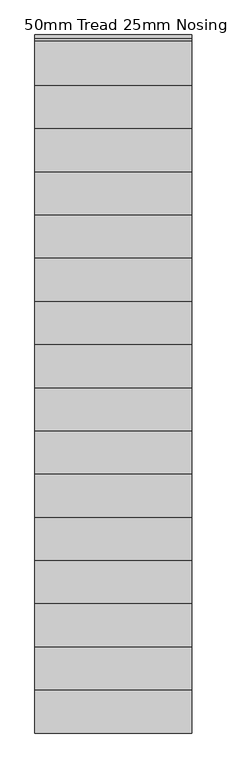
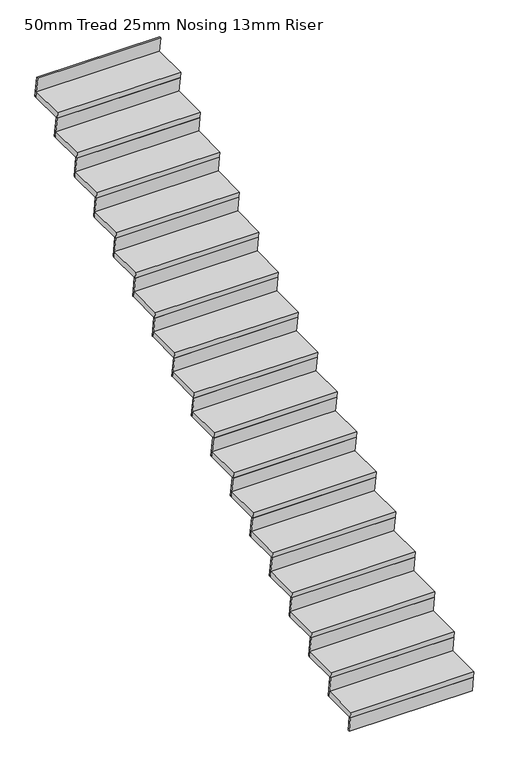
"""IFC4 building model written with IfcOpenShell, lengths in millimetres: stair flight geometry, 50mm Tread 25mm Nosing 13mm Riser."""

import ifcopenshell
import ifcopenshell.guid

model = None  # the IFC model being written
_history = None  # IfcOwnerHistory: only IFC2X3 demands one
_inside = {}  # id of a spatial element -> (the spatial element, [elements in it])
_under = {}  # id of a project, library or spatial element -> (it, [spatial elements below it])
_declared = {}  # id of a project -> (the project, [libraries it declares])
_typed = {}  # id of a type object -> (the type object, [elements of that type])
_made_of = {}  # id of a material, layer set ... -> (it, [elements and type objects made of it])


def new_model(schema):
    """Start an empty IFC model of exactly this schema.

    Asked for "IFC4X3", IfcOpenShell would pick the latest addendum, in which some entities
    have other attributes; the version numbers below select the first issue.
    IFC2X3 requires an IfcOwnerHistory on every rooted entity: one is made here for all.
    """
    global model, _history
    if schema == "IFC4X3":
        model = ifcopenshell.file(schema_version=(4, 3, 0, 0))
    else:
        model = ifcopenshell.file(schema=schema)
    _inside.clear()
    _under.clear()
    _declared.clear()
    _typed.clear()
    _made_of.clear()
    _history = None
    if model.schema == "IFC2X3":
        org = make("IfcOrganization", Name="unknown")
        user = make(
            "IfcPersonAndOrganization",
            ThePerson=make("IfcPerson", FamilyName="unknown"),
            TheOrganization=org,
        )
        app = make(
            "IfcApplication",
            ApplicationDeveloper=org,
            Version="unknown",
            ApplicationFullName="unknown",
            ApplicationIdentifier="unknown",
        )
        _history = make(
            "IfcOwnerHistory",
            OwningUser=user,
            OwningApplication=app,
            ChangeAction="ADDED",
            CreationDate=0,
        )
    return model


def make(cls, **values):
    """One entity of the class cls with the attributes given. An attribute that is None is left unset."""
    return model.create_entity(
        cls, **{name: value for name, value in values.items() if value is not None}
    )


def rooted(cls, **values):
    """An entity with a GlobalId (a new one), such as an element, a storey or a relation."""
    return make(cls, GlobalId=ifcopenshell.guid.new(), OwnerHistory=_history, **values)


def si_unit(unit_type, name, prefix=None):
    """IfcSIUnit, for example si_unit("LENGTHUNIT", "METRE", prefix="MILLI")."""
    return make("IfcSIUnit", UnitType=unit_type, Prefix=prefix, Name=name)


def assignment(units):
    """IfcUnitAssignment: the units of a project."""
    return None if units is None else make("IfcUnitAssignment", Units=units)


def point(xyz):
    """IfcCartesianPoint."""
    return None if xyz is None else make("IfcCartesianPoint", Coordinates=xyz)


def direction(xyz):
    """IfcDirection."""
    return None if xyz is None else make("IfcDirection", DirectionRatios=xyz)


def frame(location, z_axis=None, x_axis=None):
    """IfcAxis2Placement3D, a coordinate frame: its origin and axes. An axis left out is left unset."""
    return make(
        "IfcAxis2Placement3D",
        Location=point(location),
        Axis=direction(z_axis),
        RefDirection=direction(x_axis),
    )


def origin():
    """The frame at (0, 0, 0) with its axes left unset."""
    return frame((0.0, 0.0, 0.0))


def place(relative_to, where):
    """IfcLocalPlacement: puts the frame where relative to a parent placement (None: the world)."""
    return make(
        "IfcLocalPlacement", PlacementRelTo=relative_to, RelativePlacement=where
    )


def context(
    kind, dimensions, precision=None, world=None, true_north=None, identifier=None
):
    """IfcGeometricRepresentationContext, for example the 3D "Model" context."""
    return make(
        "IfcGeometricRepresentationContext",
        ContextIdentifier=identifier,
        ContextType=kind,
        CoordinateSpaceDimension=dimensions,
        Precision=precision,
        WorldCoordinateSystem=world,
        TrueNorth=true_north,
    )


def project(units=None, contexts=None):
    """IfcProject with its units and contexts."""
    return rooted(
        "IfcProject",
        Name="project",
        RepresentationContexts=contexts,
        UnitsInContext=assignment(units),
    )


def spatial(cls, under=None, at=None, **own):
    """A site, building, storey or space (cls), placed at a placement, below another one or the project."""
    s = rooted(cls, ObjectPlacement=at, **own)
    if under is not None:
        _under.setdefault(under.id(), (under, []))[1].append(s)
    return s


def polyline(points):
    """IfcPolyline through the points."""
    return make("IfcPolyline", Points=[point(p) for p in points])


def outline(outer, holes=None, kind="AREA"):
    """IfcArbitraryClosedProfileDef: a profile drawn as a closed curve; with holes, ...WithVoids."""
    if holes is None:
        return make("IfcArbitraryClosedProfileDef", ProfileType=kind, OuterCurve=outer)
    return make(
        "IfcArbitraryProfileDefWithVoids",
        ProfileType=kind,
        OuterCurve=outer,
        InnerCurves=holes,
    )


def extrude(swept, where, along, depth):
    """IfcExtrudedAreaSolid: the profile swept, set in the frame where, extruded along a direction by depth."""
    return make(
        "IfcExtrudedAreaSolid",
        SweptArea=swept,
        Position=where,
        ExtrudedDirection=direction(along),
        Depth=depth,
    )


def shape(context_of_items, identifier, shape_type, items):
    """IfcShapeRepresentation: the items that make up one representation, for example the "Body"."""
    return make(
        "IfcShapeRepresentation",
        ContextOfItems=context_of_items,
        RepresentationIdentifier=identifier,
        RepresentationType=shape_type,
        Items=items,
    )


def source(mapping_origin, context_of_items, identifier, shape_type, items):
    """IfcRepresentationMap: a shape defined once, which mapped items show again and again."""
    return make(
        "IfcRepresentationMap",
        MappingOrigin=mapping_origin,
        MappedRepresentation=shape(context_of_items, identifier, shape_type, items),
    )


def transform(
    local_origin,
    x_axis=None,
    y_axis=None,
    z_axis=None,
    scale=None,
    scale2=None,
    scale3=None,
    uniform=True,
):
    """IfcCartesianTransformationOperator3D, or its non-uniform kind. x_axis, y_axis, z_axis: its Axis1, 2, 3."""
    if uniform:
        return make(
            "IfcCartesianTransformationOperator3D",
            Axis1=direction(x_axis),
            Axis2=direction(y_axis),
            LocalOrigin=point(local_origin),
            Scale=scale,
            Axis3=direction(z_axis),
        )
    return make(
        "IfcCartesianTransformationOperator3DnonUniform",
        Axis1=direction(x_axis),
        Axis2=direction(y_axis),
        LocalOrigin=point(local_origin),
        Scale=scale,
        Axis3=direction(z_axis),
        Scale2=scale2,
        Scale3=scale3,
    )


def mapped(mapping_source, mapping_target):
    """IfcMappedItem: shows the shape of a source again, moved by a transform."""
    return make(
        "IfcMappedItem", MappingSource=mapping_source, MappingTarget=mapping_target
    )


def made_of(thing, what):
    """Note that an element or type object is made of a material, layer set ...; save() writes the relation."""
    if what is not None:
        _made_of.setdefault(what.id(), (what, []))[1].append(thing)
    return thing


def element(
    cls,
    number,
    at=None,
    inside=None,
    cuts=None,
    type_object=None,
    material=None,
    context=None,
    identifier="Body",
    shape_type=None,
    held_by="IfcProductDefinitionShape",
    body=None,
    shapes=None,
    **own,
):
    """One element of the class cls, such as IfcWall. Its Tag is "e" and its number.

    at: its placement. inside: the storey or other place that contains it. cuts: it is an
    opening in that element (IfcRelVoidsElement). A single representation is given by context,
    identifier, shape_type and body (its items); several are given by shapes. held_by: the class
    of the entity that holds the representations. save() writes the other relations.
    """
    e = rooted(cls, Tag="e%d" % number, ObjectPlacement=at, **own)
    if body is not None:
        shapes = [shape(context, identifier, shape_type, body)]
    if shapes is not None:
        e.Representation = make(held_by, Representations=shapes)
    if inside is not None:
        _inside.setdefault(inside.id(), (inside, []))[1].append(e)
    if cuts is not None:
        rooted(
            "IfcRelVoidsElement", RelatingBuildingElement=cuts, RelatedOpeningElement=e
        )
    if type_object is not None:
        _typed.setdefault(type_object.id(), (type_object, []))[1].append(e)
    return made_of(e, material)


def aggregate(whole, parts):
    """IfcRelAggregates: a whole, such as a stair, and the parts it consists of."""
    return rooted("IfcRelAggregates", RelatingObject=whole, RelatedObjects=parts)


def save(model, path):
    """Write the relations noted so far, then the file.

    IfcRelAggregates (storeys below a building ...), IfcRelContainedInSpatialStructure (elements
    in a storey), IfcRelDefinesByType, IfcRelAssociatesMaterial and IfcRelDeclares: one each for
    every whole, place, type object, material and project.
    """
    for whole, parts in _under.values():
        aggregate(whole, parts)
    for where, things in _inside.values():
        rooted(
            "IfcRelContainedInSpatialStructure",
            RelatedElements=things,
            RelatingStructure=where,
        )
    for kind, things in _typed.values():
        rooted("IfcRelDefinesByType", RelatedObjects=things, RelatingType=kind)
    for what, things in _made_of.values():
        rooted("IfcRelAssociatesMaterial", RelatedObjects=things, RelatingMaterial=what)
    for by, libraries in _declared.values():
        rooted("IfcRelDeclares", RelatingContext=by, RelatedDefinitions=libraries)
    model.write(path)


def stair_flight_50mm_tread_25mm_nosing_13mm_riser_3b40119f(model_context):
    return source(origin(), model_context, "Body", "SweptSolid", [
        extrude(outline(polyline([(-31126.6946949, 176.4705882), (-30826.6946949, 176.4705882), (-30819.6113616, 126.4705882), (-31119.6113616, 126.4705882), (-31126.6946949, 176.4705882)])), frame((121318.8827039, 0.0, 0.0), z_axis=(1.0, 0.0, 0.0), x_axis=(0.0, 1.0, 0.0)), (0.0, 0.0, 1.0), 1000.0),
        extrude(outline(polyline([(-31119.6113616, 126.4705882), (-31106.9865507, 126.4705882), (-31089.069884, 0.0), (-31101.6946949, 0.0), (-31119.6113616, 126.4705882)])), frame((121318.8827039, 0.0, 0.0), z_axis=(1.0, 0.0, 0.0), x_axis=(0.0, 1.0, 0.0)), (0.0, 0.0, 1.0), 1000.0),
        extrude(outline(polyline([(-30844.6113616, 302.9411765), (-30831.9865507, 302.9411765), (-30806.9865507, 126.4705882), (-30819.6113616, 126.4705882), (-30844.6113616, 302.9411765)])), frame((121318.8827039, 0.0, 0.0), z_axis=(1.0, 0.0, 0.0), x_axis=(0.0, 1.0, 0.0)), (0.0, 0.0, 1.0), 1000.0),
        extrude(outline(polyline([(-30851.6946949, 352.9411765), (-30551.6946949, 352.9411765), (-30544.6113616, 302.9411765), (-30844.6113616, 302.9411765), (-30851.6946949, 352.9411765)])), frame((121318.8827039, 0.0, 0.0), z_axis=(1.0, 0.0, 0.0), x_axis=(0.0, 1.0, 0.0)), (0.0, 0.0, 1.0), 1000.0),
        extrude(outline(polyline([(-30569.6113616, 479.4117647), (-30556.9865507, 479.4117647), (-30531.9865507, 302.9411765), (-30544.6113616, 302.9411765), (-30569.6113616, 479.4117647)])), frame((121318.8827039, 0.0, 0.0), z_axis=(1.0, 0.0, 0.0), x_axis=(0.0, 1.0, 0.0)), (0.0, 0.0, 1.0), 1000.0),
        extrude(outline(polyline([(-30576.6946949, 529.4117647), (-30276.6946949, 529.4117647), (-30269.6113616, 479.4117647), (-30569.6113616, 479.4117647), (-30576.6946949, 529.4117647)])), frame((121318.8827039, 0.0, 0.0), z_axis=(1.0, 0.0, 0.0), x_axis=(0.0, 1.0, 0.0)), (0.0, 0.0, 1.0), 1000.0),
        extrude(outline(polyline([(-30294.6113616, 655.8823529), (-30281.9865507, 655.8823529), (-30256.9865507, 479.4117647), (-30269.6113616, 479.4117647), (-30294.6113616, 655.8823529)])), frame((121318.8827039, 0.0, 0.0), z_axis=(1.0, 0.0, 0.0), x_axis=(0.0, 1.0, 0.0)), (0.0, 0.0, 1.0), 1000.0),
        extrude(outline(polyline([(-30301.6946949, 705.8823529), (-30001.6946949, 705.8823529), (-29994.6113616, 655.8823529), (-30294.6113616, 655.8823529), (-30301.6946949, 705.8823529)])), frame((121318.8827039, 0.0, 0.0), z_axis=(1.0, 0.0, 0.0), x_axis=(0.0, 1.0, 0.0)), (0.0, 0.0, 1.0), 1000.0),
        extrude(outline(polyline([(-30019.6113616, 832.3529412), (-30006.9865507, 832.3529412), (-29981.9865507, 655.8823529), (-29994.6113616, 655.8823529), (-30019.6113616, 832.3529412)])), frame((121318.8827039, 0.0, 0.0), z_axis=(1.0, 0.0, 0.0), x_axis=(0.0, 1.0, 0.0)), (0.0, 0.0, 1.0), 1000.0),
        extrude(outline(polyline([(-30026.6946949, 882.3529412), (-29726.6946949, 882.3529412), (-29719.6113616, 832.3529412), (-30019.6113616, 832.3529412), (-30026.6946949, 882.3529412)])), frame((121318.8827039, 0.0, 0.0), z_axis=(1.0, 0.0, 0.0), x_axis=(0.0, 1.0, 0.0)), (0.0, 0.0, 1.0), 1000.0),
        extrude(outline(polyline([(-29744.6113616, 1008.8235294), (-29731.9865507, 1008.8235294), (-29706.9865507, 832.3529412), (-29719.6113616, 832.3529412), (-29744.6113616, 1008.8235294)])), frame((121318.8827039, 0.0, 0.0), z_axis=(1.0, 0.0, 0.0), x_axis=(0.0, 1.0, 0.0)), (0.0, 0.0, 1.0), 1000.0),
        extrude(outline(polyline([(-29751.6946949, 1058.8235294), (-29451.6946949, 1058.8235294), (-29444.6113616, 1008.8235294), (-29744.6113616, 1008.8235294), (-29751.6946949, 1058.8235294)])), frame((121318.8827039, 0.0, 0.0), z_axis=(1.0, 0.0, 0.0), x_axis=(0.0, 1.0, 0.0)), (0.0, 0.0, 1.0), 1000.0),
        extrude(outline(polyline([(-29469.6113616, 1185.2941176), (-29456.9865507, 1185.2941176), (-29431.9865507, 1008.8235294), (-29444.6113616, 1008.8235294), (-29469.6113616, 1185.2941176)])), frame((121318.8827039, 0.0, 0.0), z_axis=(1.0, 0.0, 0.0), x_axis=(0.0, 1.0, 0.0)), (0.0, 0.0, 1.0), 1000.0),
        extrude(outline(polyline([(-29476.6946949, 1235.2941176), (-29176.6946949, 1235.2941176), (-29169.6113616, 1185.2941176), (-29469.6113616, 1185.2941176), (-29476.6946949, 1235.2941176)])), frame((121318.8827039, 0.0, 0.0), z_axis=(1.0, 0.0, 0.0), x_axis=(0.0, 1.0, 0.0)), (0.0, 0.0, 1.0), 1000.0),
        extrude(outline(polyline([(-29194.6113616, 1361.7647059), (-29181.9865507, 1361.7647059), (-29156.9865507, 1185.2941176), (-29169.6113616, 1185.2941176), (-29194.6113616, 1361.7647059)])), frame((121318.8827039, 0.0, 0.0), z_axis=(1.0, 0.0, 0.0), x_axis=(0.0, 1.0, 0.0)), (0.0, 0.0, 1.0), 1000.0),
        extrude(outline(polyline([(-29201.6946949, 1411.7647059), (-28901.6946949, 1411.7647059), (-28894.6113616, 1361.7647059), (-29194.6113616, 1361.7647059), (-29201.6946949, 1411.7647059)])), frame((121318.8827039, 0.0, 0.0), z_axis=(1.0, 0.0, 0.0), x_axis=(0.0, 1.0, 0.0)), (0.0, 0.0, 1.0), 1000.0),
        extrude(outline(polyline([(-28919.6113616, 1538.2352941), (-28906.9865507, 1538.2352941), (-28881.9865507, 1361.7647059), (-28894.6113616, 1361.7647059), (-28919.6113616, 1538.2352941)])), frame((121318.8827039, 0.0, 0.0), z_axis=(1.0, 0.0, 0.0), x_axis=(0.0, 1.0, 0.0)), (0.0, 0.0, 1.0), 1000.0),
        extrude(outline(polyline([(-28926.6946949, 1588.2352941), (-28626.6946949, 1588.2352941), (-28619.6113616, 1538.2352941), (-28919.6113616, 1538.2352941), (-28926.6946949, 1588.2352941)])), frame((121318.8827039, 0.0, 0.0), z_axis=(1.0, 0.0, 0.0), x_axis=(0.0, 1.0, 0.0)), (0.0, 0.0, 1.0), 1000.0),
        extrude(outline(polyline([(-28644.6113616, 1714.7058824), (-28631.9865507, 1714.7058824), (-28606.9865507, 1538.2352941), (-28619.6113616, 1538.2352941), (-28644.6113616, 1714.7058824)])), frame((121318.8827039, 0.0, 0.0), z_axis=(1.0, 0.0, 0.0), x_axis=(0.0, 1.0, 0.0)), (0.0, 0.0, 1.0), 1000.0),
        extrude(outline(polyline([(-28651.6946949, 1764.7058824), (-28351.6946949, 1764.7058824), (-28344.6113616, 1714.7058824), (-28644.6113616, 1714.7058824), (-28651.6946949, 1764.7058824)])), frame((121318.8827039, 0.0, 0.0), z_axis=(1.0, 0.0, 0.0), x_axis=(0.0, 1.0, 0.0)), (0.0, 0.0, 1.0), 1000.0),
        extrude(outline(polyline([(-28369.6113616, 1891.1764706), (-28356.9865507, 1891.1764706), (-28331.9865507, 1714.7058824), (-28344.6113616, 1714.7058824), (-28369.6113616, 1891.1764706)])), frame((121318.8827039, 0.0, 0.0), z_axis=(1.0, 0.0, 0.0), x_axis=(0.0, 1.0, 0.0)), (0.0, 0.0, 1.0), 1000.0),
        extrude(outline(polyline([(-28376.6946949, 1941.1764706), (-28076.6946949, 1941.1764706), (-28069.6113616, 1891.1764706), (-28369.6113616, 1891.1764706), (-28376.6946949, 1941.1764706)])), frame((121318.8827039, 0.0, 0.0), z_axis=(1.0, 0.0, 0.0), x_axis=(0.0, 1.0, 0.0)), (0.0, 0.0, 1.0), 1000.0),
        extrude(outline(polyline([(-28094.6113616, 2067.6470588), (-28081.9865507, 2067.6470588), (-28056.9865507, 1891.1764706), (-28069.6113616, 1891.1764706), (-28094.6113616, 2067.6470588)])), frame((121318.8827039, 0.0, 0.0), z_axis=(1.0, 0.0, 0.0), x_axis=(0.0, 1.0, 0.0)), (0.0, 0.0, 1.0), 1000.0),
        extrude(outline(polyline([(-28101.6946949, 2117.6470588), (-27801.6946949, 2117.6470588), (-27794.6113616, 2067.6470588), (-28094.6113616, 2067.6470588), (-28101.6946949, 2117.6470588)])), frame((121318.8827039, 0.0, 0.0), z_axis=(1.0, 0.0, 0.0), x_axis=(0.0, 1.0, 0.0)), (0.0, 0.0, 1.0), 1000.0),
        extrude(outline(polyline([(-27819.6113616, 2244.1176471), (-27806.9865507, 2244.1176471), (-27781.9865507, 2067.6470588), (-27794.6113616, 2067.6470588), (-27819.6113616, 2244.1176471)])), frame((121318.8827039, 0.0, 0.0), z_axis=(1.0, 0.0, 0.0), x_axis=(0.0, 1.0, 0.0)), (0.0, 0.0, 1.0), 1000.0),
        extrude(outline(polyline([(-27826.6946949, 2294.1176471), (-27526.6946949, 2294.1176471), (-27519.6113616, 2244.1176471), (-27819.6113616, 2244.1176471), (-27826.6946949, 2294.1176471)])), frame((121318.8827039, 0.0, 0.0), z_axis=(1.0, 0.0, 0.0), x_axis=(0.0, 1.0, 0.0)), (0.0, 0.0, 1.0), 1000.0),
        extrude(outline(polyline([(-27544.6113616, 2420.5882353), (-27531.9865507, 2420.5882353), (-27506.9865507, 2244.1176471), (-27519.6113616, 2244.1176471), (-27544.6113616, 2420.5882353)])), frame((121318.8827039, 0.0, 0.0), z_axis=(1.0, 0.0, 0.0), x_axis=(0.0, 1.0, 0.0)), (0.0, 0.0, 1.0), 1000.0),
        extrude(outline(polyline([(-27551.6946949, 2470.5882353), (-27251.6946949, 2470.5882353), (-27244.6113616, 2420.5882353), (-27544.6113616, 2420.5882353), (-27551.6946949, 2470.5882353)])), frame((121318.8827039, 0.0, 0.0), z_axis=(1.0, 0.0, 0.0), x_axis=(0.0, 1.0, 0.0)), (0.0, 0.0, 1.0), 1000.0),
        extrude(outline(polyline([(-27269.6113616, 2597.0588235), (-27256.9865507, 2597.0588235), (-27231.9865507, 2420.5882353), (-27244.6113616, 2420.5882353), (-27269.6113616, 2597.0588235)])), frame((121318.8827039, 0.0, 0.0), z_axis=(1.0, 0.0, 0.0), x_axis=(0.0, 1.0, 0.0)), (0.0, 0.0, 1.0), 1000.0),
        extrude(outline(polyline([(-27276.6946949, 2647.0588235), (-26976.6946949, 2647.0588235), (-26969.6113616, 2597.0588235), (-27269.6113616, 2597.0588235), (-27276.6946949, 2647.0588235)])), frame((121318.8827039, 0.0, 0.0), z_axis=(1.0, 0.0, 0.0), x_axis=(0.0, 1.0, 0.0)), (0.0, 0.0, 1.0), 1000.0),
        extrude(outline(polyline([(-26994.6113616, 2773.5294118), (-26981.9865507, 2773.5294118), (-26956.9865507, 2597.0588235), (-26969.6113616, 2597.0588235), (-26994.6113616, 2773.5294118)])), frame((121318.8827039, 0.0, 0.0), z_axis=(1.0, 0.0, 0.0), x_axis=(0.0, 1.0, 0.0)), (0.0, 0.0, 1.0), 1000.0),
        extrude(outline(polyline([(-26719.6113616, 2950.0), (-26706.9865507, 2950.0), (-26681.9865507, 2773.5294118), (-26694.6113616, 2773.5294118), (-26719.6113616, 2950.0)])), frame((121318.8827039, 0.0, 0.0), z_axis=(1.0, 0.0, 0.0), x_axis=(0.0, 1.0, 0.0)), (0.0, 0.0, 1.0), 1000.0),
        extrude(outline(polyline([(-27001.6946949, 2823.5294118), (-26701.6946949, 2823.5294118), (-26694.6113616, 2773.5294118), (-26994.6113616, 2773.5294118), (-27001.6946949, 2823.5294118)])), frame((121318.8827039, 0.0, 0.0), z_axis=(1.0, 0.0, 0.0), x_axis=(0.0, 1.0, 0.0)), (0.0, 0.0, 1.0), 1000.0),
    ])


if __name__ == "__main__":
    model = new_model("IFC4")
    model_context = context("Model", 3, world=origin())
    ifc_project = project(units=[si_unit("LENGTHUNIT", "METRE", prefix="MILLI")], contexts=[model_context])
    site = spatial("IfcSite", under=ifc_project)
    building = spatial("IfcBuilding", under=site)
    placement = place(None, origin())
    stair_flight_50mm_tread_25mm_nosing_13mm_riser_shape = stair_flight_50mm_tread_25mm_nosing_13mm_riser_3b40119f(model_context)
    element("IfcStairFlight", 1, ObjectType="50mm Tread 25mm Nosing 13mm Riser", at=placement, inside=building, context=model_context, shape_type="MappedRepresentation", body=[
        mapped(stair_flight_50mm_tread_25mm_nosing_13mm_riser_shape, transform((0.0, 0.0, 0.0), x_axis=(1.0, 0.0, 0.0), y_axis=(0.0, 1.0, 0.0), z_axis=(0.0, 0.0, 1.0))),
    ])
    save(model, "model.ifc")

# Revit data of these elements
# Project information
#   Project Issue Date = "Issue Date"
#   Project Status = "Project  Status"
#   Client Name = "Owner"
#   Project Address = "## Street\nCity, State  Zip"
#   Project Name = "Project Name"
#   Project Number = "Project  Number"
